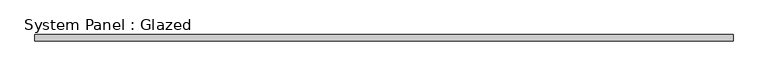
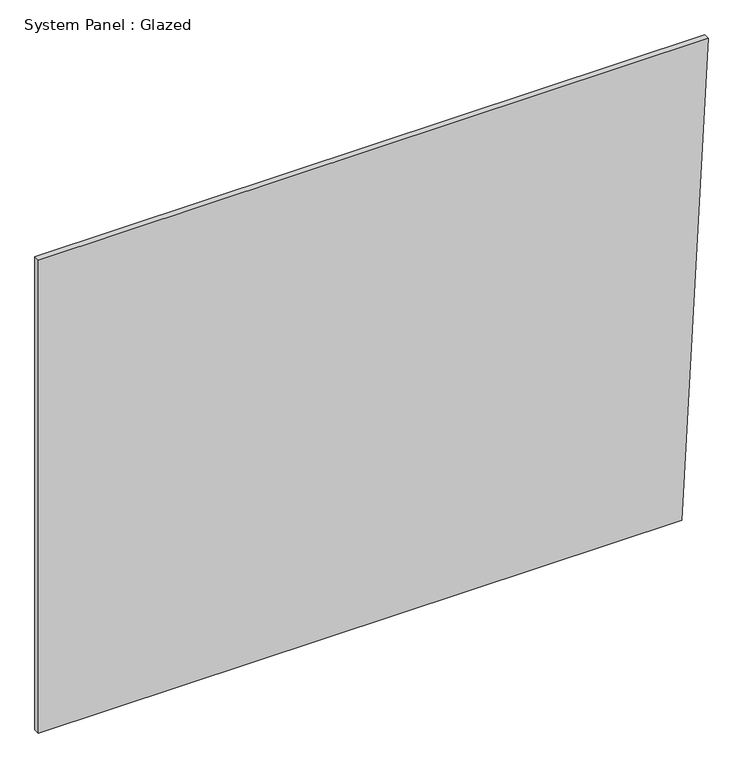
"""IFC4 building model written with IfcOpenShell, lengths in millimetres: plate geometry, System Panel : Glazed."""

from ifc_helpers import new_model, si_unit, frame, origin, place, context, project, spatial, polyline, outline, extrude, source, transform, mapped, element, save


def system_panel_glazed_3b2a3880(model_context):
    return source(origin(), model_context, "Body", "SweptSolid", [
        extrude(outline(polyline([(0.0, -1396.3622347), (0.0, 1287.2219516), (2085.3785982, 1396.3622347), (2085.3785982, -1396.3622347), (0.0, -1396.3622347)])), frame((0.0, -44.45, 0.0), z_axis=(0.0, 1.0, 0.0), x_axis=(0.0, 0.0, 1.0)), (0.0, 0.0, 1.0), 25.4),
    ])


if __name__ == "__main__":
    model = new_model("IFC4")
    model_context = context("Model", 3, world=origin())
    ifc_project = project(units=[si_unit("LENGTHUNIT", "METRE", prefix="MILLI")], contexts=[model_context])
    site = spatial("IfcSite", under=ifc_project)
    building = spatial("IfcBuilding", under=site)
    placement = place(None, origin())
    system_panel_glazed_shape = system_panel_glazed_3b2a3880(model_context)
    element("IfcPlate", 1, ObjectType="System Panel : Glazed", at=placement, inside=building, context=model_context, shape_type="MappedRepresentation", body=[
        mapped(system_panel_glazed_shape, transform((0.0, 0.0, 0.0), x_axis=(1.0, 0.0, 0.0), y_axis=(0.0, 1.0, 0.0), z_axis=(0.0, 0.0, 1.0))),
    ])
    save(model, "model.ifc")

# Revit data of these elements
# Type "System Panel : Glazed"
#   Construction Type Id = "GSP4R"
#   Analytic Construction = "1/8 in Pilkington single glazing"
#   Visual Light Transmittance = 0.9
#   Solar Heat Gain Coefficient = 0.86
#   Heat Transfer Coefficient (U) = 1.18115 BTU/(h·ft²·°F)
#   Define Thermal Properties by = 1
# Element 1 (IfcPlate, "System Panel : Glazed")
#   Materials on its faces: "Glass"
# Materials
#   "Glass": class "Glass", colour RGB 0 128 192, transparency 0.75, Description = "Soda Lime Glass", Cost = 0
